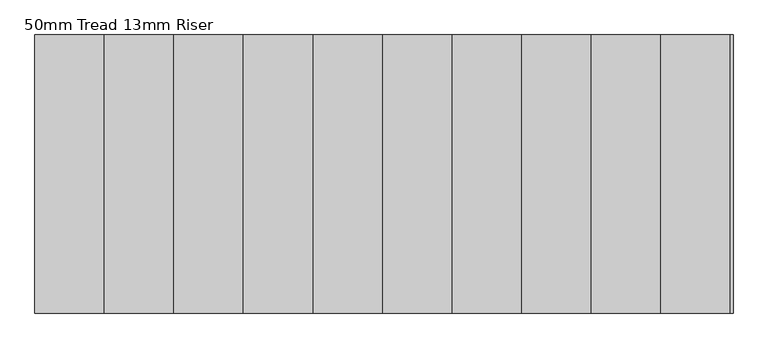
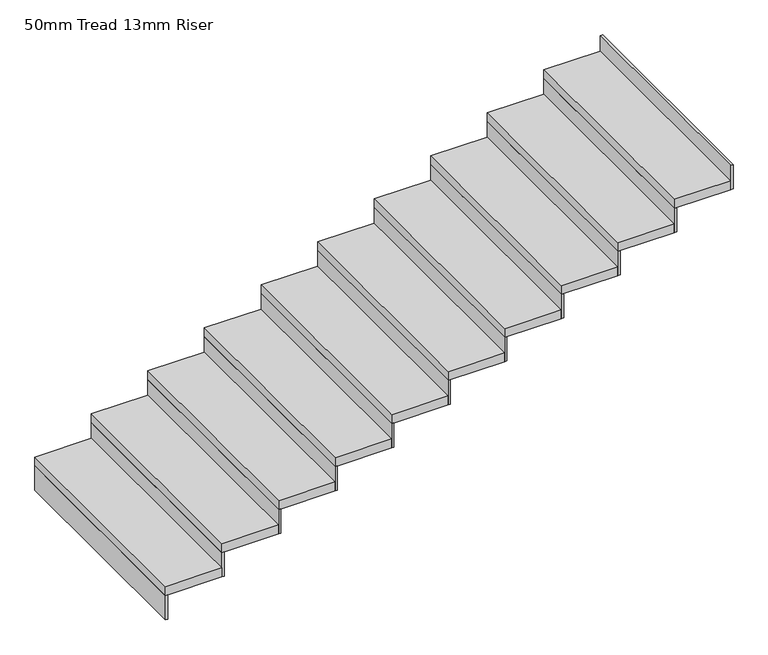
"""IFC4 building model written with IfcOpenShell, lengths in millimetres: stair flight geometry, 50mm Tread 13mm Riser."""

from ifc_helpers import new_model, si_unit, frame, origin, place, context, project, spatial, polyline, outline, extrude, source, transform, mapped, element, save


def stair_flight_50mm_tread_13mm_riser_9a58d048(model_context):
    return source(origin(), model_context, "Body", "SweptSolid", [
        extrude(outline(polyline([(-10015.2499729, -6081.4588442), (-10027.7499729, -6081.4588442), (-10027.7499729, -4881.4588442), (-10015.2499729, -4881.4588442), (-10015.2499729, -6081.4588442)])), frame((0.0, 0.0, 1450.0), z_axis=(0.0, 0.0, 1.0), x_axis=(1.0, 0.0, 0.0)), (0.0, 0.0, 1.0), 136.3636364),
        extrude(outline(polyline([(-9727.7499729, -4881.4588442), (-9727.7499729, -6081.4588442), (-10027.7499729, -6081.4588442), (-10027.7499729, -4881.4588442), (-9727.7499729, -4881.4588442)])), frame((0.0, 0.0, 1586.3636364), z_axis=(0.0, 0.0, 1.0), x_axis=(1.0, 0.0, 0.0)), (0.0, 0.0, 1.0), 50.0),
        extrude(outline(polyline([(-9715.2499729, -6081.4588442), (-9727.7499729, -6081.4588442), (-9727.7499729, -4881.4588442), (-9715.2499729, -4881.4588442), (-9715.2499729, -6081.4588442)])), frame((0.0, 0.0, 1586.3636364), z_axis=(0.0, 0.0, 1.0), x_axis=(1.0, 0.0, 0.0)), (0.0, 0.0, 1.0), 136.3636364),
        extrude(outline(polyline([(-9427.7499729, -4881.4588442), (-9427.7499729, -6081.4588442), (-9727.7499729, -6081.4588442), (-9727.7499729, -4881.4588442), (-9427.7499729, -4881.4588442)])), frame((0.0, 0.0, 1722.7272727), z_axis=(0.0, 0.0, 1.0), x_axis=(1.0, 0.0, 0.0)), (0.0, 0.0, 1.0), 50.0),
        extrude(outline(polyline([(-9415.2499729, -6081.4588442), (-9427.7499729, -6081.4588442), (-9427.7499729, -4881.4588442), (-9415.2499729, -4881.4588442), (-9415.2499729, -6081.4588442)])), frame((0.0, 0.0, 1722.7272727), z_axis=(0.0, 0.0, 1.0), x_axis=(1.0, 0.0, 0.0)), (0.0, 0.0, 1.0), 136.3636364),
        extrude(outline(polyline([(-9127.7499729, -4881.4588442), (-9127.7499729, -6081.4588442), (-9427.7499729, -6081.4588442), (-9427.7499729, -4881.4588442), (-9127.7499729, -4881.4588442)])), frame((0.0, 0.0, 1859.0909091), z_axis=(0.0, 0.0, 1.0), x_axis=(1.0, 0.0, 0.0)), (0.0, 0.0, 1.0), 50.0),
        extrude(outline(polyline([(-9115.2499729, -6081.4588442), (-9127.7499729, -6081.4588442), (-9127.7499729, -4881.4588442), (-9115.2499729, -4881.4588442), (-9115.2499729, -6081.4588442)])), frame((0.0, 0.0, 1859.0909091), z_axis=(0.0, 0.0, 1.0), x_axis=(1.0, 0.0, 0.0)), (0.0, 0.0, 1.0), 136.3636364),
        extrude(outline(polyline([(-8827.7499729, -4881.4588442), (-8827.7499729, -6081.4588442), (-9127.7499729, -6081.4588442), (-9127.7499729, -4881.4588442), (-8827.7499729, -4881.4588442)])), frame((0.0, 0.0, 1995.4545455), z_axis=(0.0, 0.0, 1.0), x_axis=(1.0, 0.0, 0.0)), (0.0, 0.0, 1.0), 50.0),
        extrude(outline(polyline([(-8815.2499729, -6081.4588442), (-8827.7499729, -6081.4588442), (-8827.7499729, -4881.4588442), (-8815.2499729, -4881.4588442), (-8815.2499729, -6081.4588442)])), frame((0.0, 0.0, 1995.4545455), z_axis=(0.0, 0.0, 1.0), x_axis=(1.0, 0.0, 0.0)), (0.0, 0.0, 1.0), 136.3636364),
        extrude(outline(polyline([(-8527.7499729, -4881.4588442), (-8527.7499729, -6081.4588442), (-8827.7499729, -6081.4588442), (-8827.7499729, -4881.4588442), (-8527.7499729, -4881.4588442)])), frame((0.0, 0.0, 2131.8181818), z_axis=(0.0, 0.0, 1.0), x_axis=(1.0, 0.0, 0.0)), (0.0, 0.0, 1.0), 50.0),
        extrude(outline(polyline([(-8515.2499729, -6081.4588442), (-8527.7499729, -6081.4588442), (-8527.7499729, -4881.4588442), (-8515.2499729, -4881.4588442), (-8515.2499729, -6081.4588442)])), frame((0.0, 0.0, 2131.8181818), z_axis=(0.0, 0.0, 1.0), x_axis=(1.0, 0.0, 0.0)), (0.0, 0.0, 1.0), 136.3636364),
        extrude(outline(polyline([(-8227.7499729, -4881.4588442), (-8227.7499729, -6081.4588442), (-8527.7499729, -6081.4588442), (-8527.7499729, -4881.4588442), (-8227.7499729, -4881.4588442)])), frame((0.0, 0.0, 2268.1818182), z_axis=(0.0, 0.0, 1.0), x_axis=(1.0, 0.0, 0.0)), (0.0, 0.0, 1.0), 50.0),
        extrude(outline(polyline([(-8215.2499729, -6081.4588442), (-8227.7499729, -6081.4588442), (-8227.7499729, -4881.4588442), (-8215.2499729, -4881.4588442), (-8215.2499729, -6081.4588442)])), frame((0.0, 0.0, 2268.1818182), z_axis=(0.0, 0.0, 1.0), x_axis=(1.0, 0.0, 0.0)), (0.0, 0.0, 1.0), 136.3636364),
        extrude(outline(polyline([(-7927.7499729, -4881.4588442), (-7927.7499729, -6081.4588442), (-8227.7499729, -6081.4588442), (-8227.7499729, -4881.4588442), (-7927.7499729, -4881.4588442)])), frame((0.0, 0.0, 2404.5454545), z_axis=(0.0, 0.0, 1.0), x_axis=(1.0, 0.0, 0.0)), (0.0, 0.0, 1.0), 50.0),
        extrude(outline(polyline([(-7915.2499729, -6081.4588442), (-7927.7499729, -6081.4588442), (-7927.7499729, -4881.4588442), (-7915.2499729, -4881.4588442), (-7915.2499729, -6081.4588442)])), frame((0.0, 0.0, 2404.5454545), z_axis=(0.0, 0.0, 1.0), x_axis=(1.0, 0.0, 0.0)), (0.0, 0.0, 1.0), 136.3636364),
        extrude(outline(polyline([(-7627.7499729, -4881.4588442), (-7627.7499729, -6081.4588442), (-7927.7499729, -6081.4588442), (-7927.7499729, -4881.4588442), (-7627.7499729, -4881.4588442)])), frame((0.0, 0.0, 2540.9090909), z_axis=(0.0, 0.0, 1.0), x_axis=(1.0, 0.0, 0.0)), (0.0, 0.0, 1.0), 50.0),
        extrude(outline(polyline([(-7615.2499729, -6081.4588442), (-7627.7499729, -6081.4588442), (-7627.7499729, -4881.4588442), (-7615.2499729, -4881.4588442), (-7615.2499729, -6081.4588442)])), frame((0.0, 0.0, 2540.9090909), z_axis=(0.0, 0.0, 1.0), x_axis=(1.0, 0.0, 0.0)), (0.0, 0.0, 1.0), 136.3636364),
        extrude(outline(polyline([(-7327.7499729, -4881.4588442), (-7327.7499729, -6081.4588442), (-7627.7499729, -6081.4588442), (-7627.7499729, -4881.4588442), (-7327.7499729, -4881.4588442)])), frame((0.0, 0.0, 2677.2727273), z_axis=(0.0, 0.0, 1.0), x_axis=(1.0, 0.0, 0.0)), (0.0, 0.0, 1.0), 50.0),
        extrude(outline(polyline([(-7315.2499729, -6081.4588442), (-7327.7499729, -6081.4588442), (-7327.7499729, -4881.4588442), (-7315.2499729, -4881.4588442), (-7315.2499729, -6081.4588442)])), frame((0.0, 0.0, 2677.2727273), z_axis=(0.0, 0.0, 1.0), x_axis=(1.0, 0.0, 0.0)), (0.0, 0.0, 1.0), 136.3636364),
        extrude(outline(polyline([(-7015.2499729, -6081.4588442), (-7027.7499729, -6081.4588442), (-7027.7499729, -4881.4588442), (-7015.2499729, -4881.4588442), (-7015.2499729, -6081.4588442)])), frame((0.0, 0.0, 2813.6363636), z_axis=(0.0, 0.0, 1.0), x_axis=(1.0, 0.0, 0.0)), (0.0, 0.0, 1.0), 136.3636364),
        extrude(outline(polyline([(-7027.7499729, -4881.4588442), (-7027.7499729, -6081.4588442), (-7327.7499729, -6081.4588442), (-7327.7499729, -4881.4588442), (-7027.7499729, -4881.4588442)])), frame((0.0, 0.0, 2813.6363636), z_axis=(0.0, 0.0, 1.0), x_axis=(1.0, 0.0, 0.0)), (0.0, 0.0, 1.0), 50.0),
    ])


if __name__ == "__main__":
    model = new_model("IFC4")
    model_context = context("Model", 3, world=origin())
    ifc_project = project(units=[si_unit("LENGTHUNIT", "METRE", prefix="MILLI")], contexts=[model_context])
    site = spatial("IfcSite", under=ifc_project)
    building = spatial("IfcBuilding", under=site)
    placement = place(None, origin())
    stair_flight_50mm_tread_13mm_riser_shape = stair_flight_50mm_tread_13mm_riser_9a58d048(model_context)
    element("IfcStairFlight", 1, ObjectType="50mm Tread 13mm Riser", at=placement, inside=building, context=model_context, shape_type="MappedRepresentation", body=[
        mapped(stair_flight_50mm_tread_13mm_riser_shape, transform((0.0, 0.0, 0.0), x_axis=(1.0, 0.0, 0.0), y_axis=(0.0, 1.0, 0.0), z_axis=(0.0, 0.0, 1.0))),
    ])
    save(model, "model.ifc")
